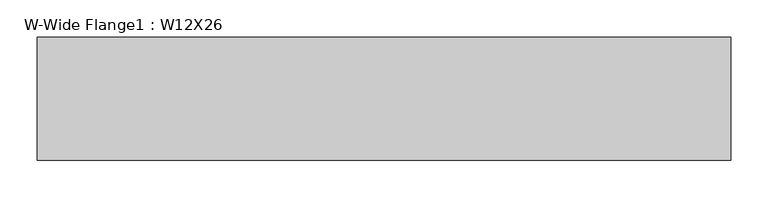
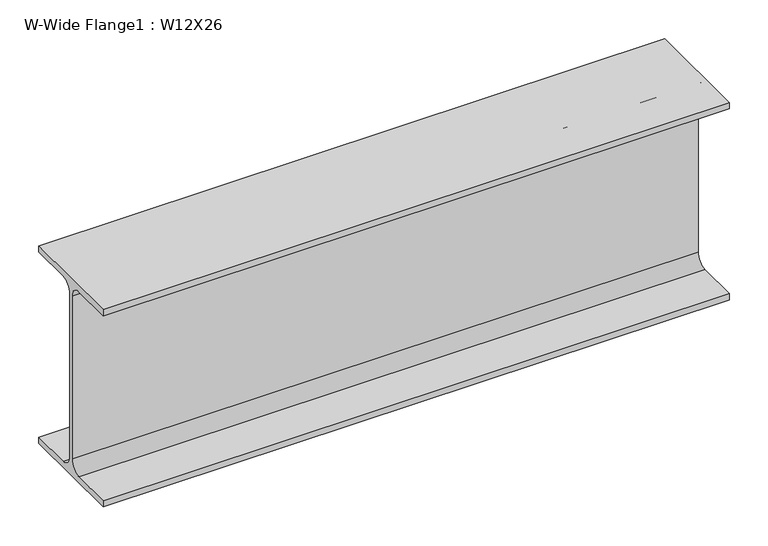
"""IFC4 building model written with IfcOpenShell, lengths in millimetres: beam geometry, W-Wide Flange1 : W12X26."""

import ifcopenshell
import ifcopenshell.guid

model = None  # the IFC model being written
_history = None  # IfcOwnerHistory: only IFC2X3 demands one
_inside = {}  # id of a spatial element -> (the spatial element, [elements in it])
_under = {}  # id of a project, library or spatial element -> (it, [spatial elements below it])
_declared = {}  # id of a project -> (the project, [libraries it declares])
_typed = {}  # id of a type object -> (the type object, [elements of that type])
_made_of = {}  # id of a material, layer set ... -> (it, [elements and type objects made of it])


def new_model(schema):
    """Start an empty IFC model of exactly this schema.

    Asked for "IFC4X3", IfcOpenShell would pick the latest addendum, in which some entities
    have other attributes; the version numbers below select the first issue.
    IFC2X3 requires an IfcOwnerHistory on every rooted entity: one is made here for all.
    """
    global model, _history
    if schema == "IFC4X3":
        model = ifcopenshell.file(schema_version=(4, 3, 0, 0))
    else:
        model = ifcopenshell.file(schema=schema)
    _inside.clear()
    _under.clear()
    _declared.clear()
    _typed.clear()
    _made_of.clear()
    _history = None
    if model.schema == "IFC2X3":
        org = make("IfcOrganization", Name="unknown")
        user = make(
            "IfcPersonAndOrganization",
            ThePerson=make("IfcPerson", FamilyName="unknown"),
            TheOrganization=org,
        )
        app = make(
            "IfcApplication",
            ApplicationDeveloper=org,
            Version="unknown",
            ApplicationFullName="unknown",
            ApplicationIdentifier="unknown",
        )
        _history = make(
            "IfcOwnerHistory",
            OwningUser=user,
            OwningApplication=app,
            ChangeAction="ADDED",
            CreationDate=0,
        )
    return model


def make(cls, **values):
    """One entity of the class cls with the attributes given. An attribute that is None is left unset."""
    return model.create_entity(
        cls, **{name: value for name, value in values.items() if value is not None}
    )


def rooted(cls, **values):
    """An entity with a GlobalId (a new one), such as an element, a storey or a relation."""
    return make(cls, GlobalId=ifcopenshell.guid.new(), OwnerHistory=_history, **values)


def si_unit(unit_type, name, prefix=None):
    """IfcSIUnit, for example si_unit("LENGTHUNIT", "METRE", prefix="MILLI")."""
    return make("IfcSIUnit", UnitType=unit_type, Prefix=prefix, Name=name)


def assignment(units):
    """IfcUnitAssignment: the units of a project."""
    return None if units is None else make("IfcUnitAssignment", Units=units)


def point(xyz):
    """IfcCartesianPoint."""
    return None if xyz is None else make("IfcCartesianPoint", Coordinates=xyz)


def direction(xyz):
    """IfcDirection."""
    return None if xyz is None else make("IfcDirection", DirectionRatios=xyz)


def frame(location, z_axis=None, x_axis=None):
    """IfcAxis2Placement3D, a coordinate frame: its origin and axes. An axis left out is left unset."""
    return make(
        "IfcAxis2Placement3D",
        Location=point(location),
        Axis=direction(z_axis),
        RefDirection=direction(x_axis),
    )


def frame_2d(location, x_axis=None):
    """IfcAxis2Placement2D, a coordinate frame in the plane: its origin and x axis."""
    return make(
        "IfcAxis2Placement2D", Location=point(location), RefDirection=direction(x_axis)
    )


def origin():
    """The frame at (0, 0, 0) with its axes left unset."""
    return frame((0.0, 0.0, 0.0))


def place(relative_to, where):
    """IfcLocalPlacement: puts the frame where relative to a parent placement (None: the world)."""
    return make(
        "IfcLocalPlacement", PlacementRelTo=relative_to, RelativePlacement=where
    )


def context(
    kind, dimensions, precision=None, world=None, true_north=None, identifier=None
):
    """IfcGeometricRepresentationContext, for example the 3D "Model" context."""
    return make(
        "IfcGeometricRepresentationContext",
        ContextIdentifier=identifier,
        ContextType=kind,
        CoordinateSpaceDimension=dimensions,
        Precision=precision,
        WorldCoordinateSystem=world,
        TrueNorth=true_north,
    )


def project(units=None, contexts=None):
    """IfcProject with its units and contexts."""
    return rooted(
        "IfcProject",
        Name="project",
        RepresentationContexts=contexts,
        UnitsInContext=assignment(units),
    )


def spatial(cls, under=None, at=None, **own):
    """A site, building, storey or space (cls), placed at a placement, below another one or the project."""
    s = rooted(cls, ObjectPlacement=at, **own)
    if under is not None:
        _under.setdefault(under.id(), (under, []))[1].append(s)
    return s


def polyline(points):
    """IfcPolyline through the points."""
    return make("IfcPolyline", Points=[point(p) for p in points])


def circle_curve(where, radius):
    """IfcCircle in the frame where."""
    return make("IfcCircle", Position=where, Radius=radius)


def trimmed(basis, trim1, trim2, sense, master):
    """IfcTrimmedCurve: the piece of a basis curve between two trims."""
    return make(
        "IfcTrimmedCurve",
        BasisCurve=basis,
        Trim1=trim1,
        Trim2=trim2,
        SenseAgreement=sense,
        MasterRepresentation=master,
    )


def segment(curve, same_sense, transition):
    """IfcCompositeCurveSegment."""
    return make(
        "IfcCompositeCurveSegment",
        Transition=transition,
        SameSense=same_sense,
        ParentCurve=curve,
    )


def composite_curve(segments, self_intersect=None):
    """IfcCompositeCurve: segments joined end to end."""
    return make("IfcCompositeCurve", Segments=segments, SelfIntersect=self_intersect)


def outline(outer, holes=None, kind="AREA"):
    """IfcArbitraryClosedProfileDef: a profile drawn as a closed curve; with holes, ...WithVoids."""
    if holes is None:
        return make("IfcArbitraryClosedProfileDef", ProfileType=kind, OuterCurve=outer)
    return make(
        "IfcArbitraryProfileDefWithVoids",
        ProfileType=kind,
        OuterCurve=outer,
        InnerCurves=holes,
    )


def extrude(swept, where, along, depth):
    """IfcExtrudedAreaSolid: the profile swept, set in the frame where, extruded along a direction by depth."""
    return make(
        "IfcExtrudedAreaSolid",
        SweptArea=swept,
        Position=where,
        ExtrudedDirection=direction(along),
        Depth=depth,
    )


def shape(context_of_items, identifier, shape_type, items):
    """IfcShapeRepresentation: the items that make up one representation, for example the "Body"."""
    return make(
        "IfcShapeRepresentation",
        ContextOfItems=context_of_items,
        RepresentationIdentifier=identifier,
        RepresentationType=shape_type,
        Items=items,
    )


def source(mapping_origin, context_of_items, identifier, shape_type, items):
    """IfcRepresentationMap: a shape defined once, which mapped items show again and again."""
    return make(
        "IfcRepresentationMap",
        MappingOrigin=mapping_origin,
        MappedRepresentation=shape(context_of_items, identifier, shape_type, items),
    )


def transform(
    local_origin,
    x_axis=None,
    y_axis=None,
    z_axis=None,
    scale=None,
    scale2=None,
    scale3=None,
    uniform=True,
):
    """IfcCartesianTransformationOperator3D, or its non-uniform kind. x_axis, y_axis, z_axis: its Axis1, 2, 3."""
    if uniform:
        return make(
            "IfcCartesianTransformationOperator3D",
            Axis1=direction(x_axis),
            Axis2=direction(y_axis),
            LocalOrigin=point(local_origin),
            Scale=scale,
            Axis3=direction(z_axis),
        )
    return make(
        "IfcCartesianTransformationOperator3DnonUniform",
        Axis1=direction(x_axis),
        Axis2=direction(y_axis),
        LocalOrigin=point(local_origin),
        Scale=scale,
        Axis3=direction(z_axis),
        Scale2=scale2,
        Scale3=scale3,
    )


def mapped(mapping_source, mapping_target):
    """IfcMappedItem: shows the shape of a source again, moved by a transform."""
    return make(
        "IfcMappedItem", MappingSource=mapping_source, MappingTarget=mapping_target
    )


def made_of(thing, what):
    """Note that an element or type object is made of a material, layer set ...; save() writes the relation."""
    if what is not None:
        _made_of.setdefault(what.id(), (what, []))[1].append(thing)
    return thing


def element(
    cls,
    number,
    at=None,
    inside=None,
    cuts=None,
    type_object=None,
    material=None,
    context=None,
    identifier="Body",
    shape_type=None,
    held_by="IfcProductDefinitionShape",
    body=None,
    shapes=None,
    **own,
):
    """One element of the class cls, such as IfcWall. Its Tag is "e" and its number.

    at: its placement. inside: the storey or other place that contains it. cuts: it is an
    opening in that element (IfcRelVoidsElement). A single representation is given by context,
    identifier, shape_type and body (its items); several are given by shapes. held_by: the class
    of the entity that holds the representations. save() writes the other relations.
    """
    e = rooted(cls, Tag="e%d" % number, ObjectPlacement=at, **own)
    if body is not None:
        shapes = [shape(context, identifier, shape_type, body)]
    if shapes is not None:
        e.Representation = make(held_by, Representations=shapes)
    if inside is not None:
        _inside.setdefault(inside.id(), (inside, []))[1].append(e)
    if cuts is not None:
        rooted(
            "IfcRelVoidsElement", RelatingBuildingElement=cuts, RelatedOpeningElement=e
        )
    if type_object is not None:
        _typed.setdefault(type_object.id(), (type_object, []))[1].append(e)
    return made_of(e, material)


def aggregate(whole, parts):
    """IfcRelAggregates: a whole, such as a stair, and the parts it consists of."""
    return rooted("IfcRelAggregates", RelatingObject=whole, RelatedObjects=parts)


def save(model, path):
    """Write the relations noted so far, then the file.

    IfcRelAggregates (storeys below a building ...), IfcRelContainedInSpatialStructure (elements
    in a storey), IfcRelDefinesByType, IfcRelAssociatesMaterial and IfcRelDeclares: one each for
    every whole, place, type object, material and project.
    """
    for whole, parts in _under.values():
        aggregate(whole, parts)
    for where, things in _inside.values():
        rooted(
            "IfcRelContainedInSpatialStructure",
            RelatedElements=things,
            RelatingStructure=where,
        )
    for kind, things in _typed.values():
        rooted("IfcRelDefinesByType", RelatedObjects=things, RelatingType=kind)
    for what, things in _made_of.values():
        rooted("IfcRelAssociatesMaterial", RelatedObjects=things, RelatingMaterial=what)
    for by, libraries in _declared.values():
        rooted("IfcRelDeclares", RelatingContext=by, RelatedDefinitions=libraries)
    model.write(path)


def w_wide_flange1_w12x26_926f8985(model_context):
    return source(origin(), model_context, "Body", "SweptSolid", [
        extrude(outline(composite_curve([segment(polyline([(82.423, -145.288), (82.423, -154.94), (-82.423, -154.94), (-82.423, -145.288), (-20.2565, -145.288)]), True, "CONTINUOUS"), segment(trimmed(circle_curve(frame_2d((-20.2565, -127.9525)), 17.3355), [point((-20.2565, -145.288))], [point((-2.921, -127.9525))], True, "CARTESIAN"), True, "CONTINUOUS"), segment(polyline([(-2.921, -127.9525), (-2.921, 127.9525)]), True, "CONTINUOUS"), segment(trimmed(circle_curve(frame_2d((-20.2565, 127.9525)), 17.3355), [point((-2.921, 127.9525))], [point((-20.2565, 145.288))], True, "CARTESIAN"), True, "CONTINUOUS"), segment(polyline([(-20.2565, 145.288), (-82.423, 145.288), (-82.423, 154.94), (82.423, 154.94), (82.423, 145.288), (20.2565, 145.288)]), True, "CONTINUOUS"), segment(trimmed(circle_curve(frame_2d((20.2565, 127.9525)), 17.3355), [point((20.2565, 145.288))], [point((2.921, 127.9525))], True, "CARTESIAN"), True, "CONTINUOUS"), segment(polyline([(2.921, 127.9525), (2.921, -127.9525)]), True, "CONTINUOUS"), segment(trimmed(circle_curve(frame_2d((20.2565, -127.9525)), 17.3355), [point((2.921, -127.9525))], [point((20.2565, -145.288))], True, "CARTESIAN"), True, "CONTINUOUS"), segment(polyline([(20.2565, -145.288), (82.423, -145.288)]), True, "CONTINUOUS")], self_intersect=False)), frame((-454.9522119, 0.0, 0.0), z_axis=(1.0, 0.0, 0.0), x_axis=(0.0, 1.0, 0.0)), (0.0, 0.0, 1.0), 929.3640836),
    ])


if __name__ == "__main__":
    model = new_model("IFC4")
    model_context = context("Model", 3, world=origin())
    ifc_project = project(units=[si_unit("LENGTHUNIT", "METRE", prefix="MILLI")], contexts=[model_context])
    site = spatial("IfcSite", under=ifc_project)
    building = spatial("IfcBuilding", under=site)
    placement = place(None, origin())
    w_wide_flange1_w12x26_shape = w_wide_flange1_w12x26_926f8985(model_context)
    element("IfcBeam", 1, ObjectType="W-Wide Flange1 : W12X26", at=placement, inside=building, context=model_context, shape_type="MappedRepresentation", body=[
        mapped(w_wide_flange1_w12x26_shape, transform((0.0, 0.0, 0.0), x_axis=(1.0, 0.0, 0.0), y_axis=(0.0, 1.0, 0.0), z_axis=(0.0, 0.0, 1.0))),
    ])
    save(model, "model.ifc")

# Revit data of these elements
# Type "W-Wide Flange1 : W12X26"
#   Assembly Code = "B10"
#   W = 26
#   Start Extension Calculation [instance default] = 10' - 0"
#   Start Extension [instance default] = -0' - 0 1/2"
#   End Extension Calculation [instance default] = 10' - 0"
#   End Extension [instance default] = -0' - 0 1/2"
#   Length [instance default] = 5' - 0"
#   bf = 0' - 6.49"
#   d = 1' - 0.2"
#   k = 0' - 1 1/16"
#   k2 = 0' - 0.6825"
#   tf = 0' - 0.38"
#   tw = 0' - 0.23"
#   A = 0.053125 SF
#   Structural Material [instance default] = Metal - Steel - ASTM A992
# Element 1 (IfcBeam, "W-Wide Flange1 : W12X26")
#   Materials on its faces: "Metal - Steel - ASTM A992"
# Materials
#   "Metal - Steel - ASTM A992": class "Metal", colour RGB 199 199 199, transparency 0
